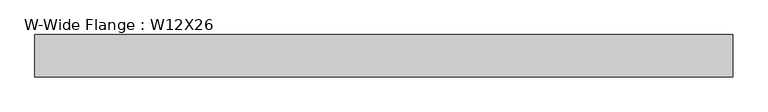
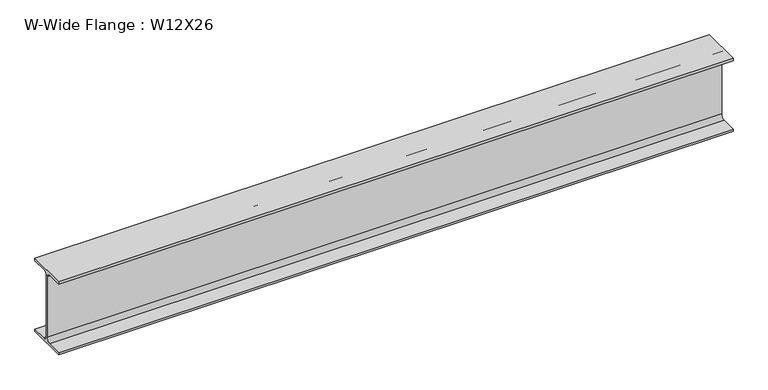
"""IFC4 building model written with IfcOpenShell, lengths in millimetres: beam geometry, W-Wide Flange : W12X26."""

from ifc_helpers import new_model, si_unit, point, frame, frame_2d, origin, place, context, project, spatial, polyline, circle_curve, trimmed, segment, composite_curve, outline, extrude, source, transform, mapped, element, save


def w_wide_flange_w12x26_563c1906(model_context):
    return source(origin(), model_context, "Body", "SweptSolid", [
        extrude(outline(composite_curve([segment(polyline([(-82.4011719, -145.5539063), (-20.2902344, -145.5539063)]), True, "CONTINUOUS"), segment(trimmed(circle_curve(frame_2d((-20.2902344, -128.190625)), 17.3632812), [point((-20.2902344, -145.5539063))], [point((-2.9269531, -128.190625))], True, "CARTESIAN"), True, "CONTINUOUS"), segment(polyline([(-2.9269531, -128.190625), (-2.9269531, 128.190625)]), True, "CONTINUOUS"), segment(trimmed(circle_curve(frame_2d((-20.2902344, 128.190625)), 17.3632812), [point((-2.9269531, 128.190625))], [point((-20.2902344, 145.5539062))], True, "CARTESIAN"), True, "CONTINUOUS"), segment(polyline([(-20.2902344, 145.5539062), (-82.4011719, 145.5539062), (-82.4011719, 155.178125), (82.4011719, 155.178125), (82.4011719, 145.5539062), (20.2902344, 145.5539062)]), True, "CONTINUOUS"), segment(trimmed(circle_curve(frame_2d((20.2902344, 128.190625)), 17.3632812), [point((20.2902344, 145.5539062))], [point((2.9269531, 128.190625))], True, "CARTESIAN"), True, "CONTINUOUS"), segment(polyline([(2.9269531, 128.190625), (2.9269531, -128.190625)]), True, "CONTINUOUS"), segment(trimmed(circle_curve(frame_2d((20.2902344, -128.190625)), 17.3632812), [point((2.9269531, -128.190625))], [point((20.2902344, -145.5539063))], True, "CARTESIAN"), True, "CONTINUOUS"), segment(polyline([(20.2902344, -145.5539063), (82.4011719, -145.5539063), (82.4011719, -155.178125), (-82.4011719, -155.178125), (-82.4011719, -145.5539063)]), True, "CONTINUOUS")], self_intersect=False)), frame((-1435.1, 0.0, 0.0), z_axis=(1.0, 0.0, 0.0), x_axis=(0.0, 1.0, 0.0)), (0.0, 0.0, 1.0), 2711.45),
    ])


if __name__ == "__main__":
    model = new_model("IFC4")
    model_context = context("Model", 3, world=origin())
    ifc_project = project(units=[si_unit("LENGTHUNIT", "METRE", prefix="MILLI")], contexts=[model_context])
    site = spatial("IfcSite", under=ifc_project)
    building = spatial("IfcBuilding", under=site)
    placement = place(None, origin())
    w_wide_flange_w12x26_shape = w_wide_flange_w12x26_563c1906(model_context)
    element("IfcBeam", 1, ObjectType="W-Wide Flange : W12X26", at=placement, inside=building, context=model_context, shape_type="MappedRepresentation", body=[
        mapped(w_wide_flange_w12x26_shape, transform((0.0, 0.0, 0.0), x_axis=(1.0, 0.0, 0.0), y_axis=(0.0, 1.0, 0.0), z_axis=(0.0, 0.0, 1.0))),
    ])
    save(model, "model.ifc")

# Revit data of these elements
# Type "W-Wide Flange : W12X26"
#   Assembly Code = "B10"
#   W = 26
#   Start Extension Calculation [instance default] = 10' - 0"
#   Start Extension [instance default] = -0' - 0 1/2"
#   End Extension Calculation [instance default] = 10' - 0"
#   End Extension [instance default] = -0' - 0 1/2"
#   Length [instance default] = 5' - 0"
#   bf = 0' - 6 125/256"
#   d = 1' - 0 7/32"
#   k = 0' - 1 1/16"
#   k2 = 0' - 0 175/256"
#   tf = 0' - 0 97/256"
#   tw = 0' - 0 59/256"
#   A = 0.05 SF
#   Beam Material [instance default] = Metal - Steel - ASTM A992
# Element 1 (IfcBeam, "W-Wide Flange : W12X26")
#   Materials on its faces: "Metal - Steel - ASTM A992"
# Materials
#   "Metal - Steel - ASTM A992": class "Metal", colour RGB 128 0 0, transparency 0
